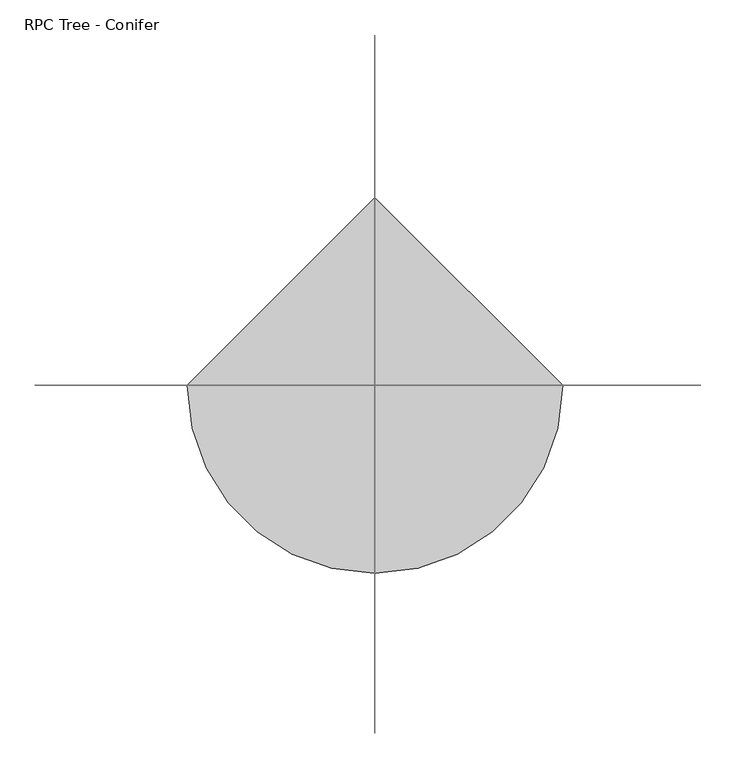
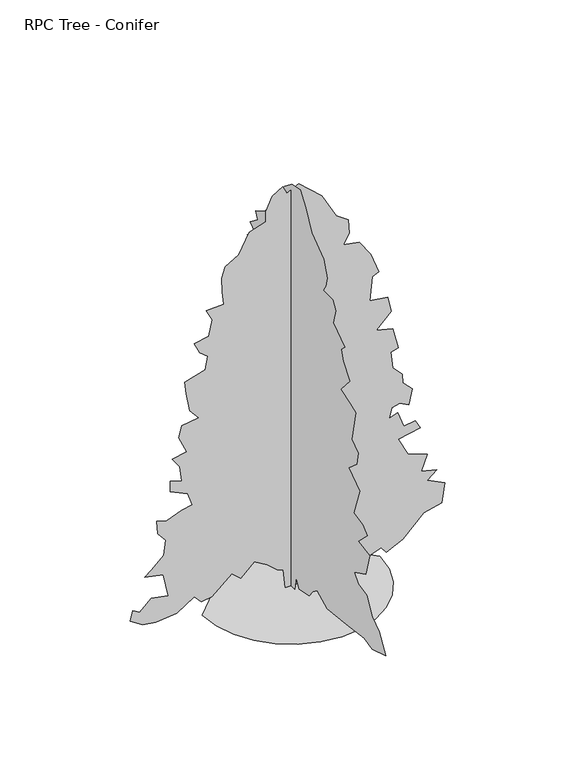
"""IFC4 building model written with IfcOpenShell, lengths in millimetres: geographic element geometry, RPC Tree - Conifer : Colorado Spruce - 4.0 Meters."""

from ifc_helpers import new_model, si_unit, origin, place, context, project, spatial, triangles, source, transform, mapped, element, save


def rpc_tree_conifer_422bf689(model_context):
    return source(origin(), model_context, "Body", "Tessellation", [
        triangles([(0.1966733, 49.8245024, 3.62e-05), (0.1966808, 76.8972503, 209.81401), (0.1966851, 110.7382534, 304.5675106), (0.1966885, 232.5655101, 236.886758), (0.1966934, 381.4650152, 175.9729979), (0.1967001, 550.6700214, 148.90025), (0.1967079, 720.3449844, 156.1022449), (0.1967054, 740.1800383, 40.6092491), (0.1967132, 862.0074858, 121.827502), (0.1967165, 991.2750315, 36.3350005), (0.1967216, 1085.3575155, 67.6820016), (0.1967296, 1268.1000675, 60.913751), (0.1967359, 1356.0849586, 142.1320039), (0.1967499, 1545.5950481, 324.872503), (0.1967463, 1430.5350655, 379.0174902), (0.1967428, 1329.0124832, 412.8600102), (0.1967383, 1234.4449997, 404.9600201), (0.1967407, 1213.9525005, 514.3825198), (0.1967447, 1241.024976, 609.1374919), (0.1967522, 1335.779948, 717.4275026), (0.1967485, 1241.024976, 737.7325132), (0.1967539, 1315.4749374, 805.4150099), (0.1967498, 1200.4174982, 839.2550228), (0.1967461, 1078.589978, 900.169982), (0.1967471, 1015.9549931, 1025.5049915), (0.1967554, 1173.3450228, 1069.3749882), (0.1967602, 1241.024976, 1130.2874765), (0.1967569, 1153.0400122, 1150.5924871), (0.1967529, 1004.1400166, 1238.5800671), (0.1967593, 1112.429991, 1292.7250179), (0.196765, 1121.189994, 1470.9574528), (0.19676, 997.3700083, 1489.0025723), (0.196756, 889.0800339, 1516.0750477), (0.1967604, 905.0550035, 1639.3949913), (0.1967674, 1036.9399767, 1676.5725185), (0.1967726, 1065.0525049, 1807.1075741), (0.1967671, 956.7625305, 1786.8025635), (0.196768, 888.3749897, 1918.5275173), (0.1967741, 963.5299953, 2010.1524479), (0.1967722, 868.7750233, 2091.3700195), (0.1967785, 963.5299953, 2159.0525162), (0.1967813, 990.6025434, 2213.197467), (0.196777, 821.3975372, 2321.4899849), (0.1967781, 801.0925266, 2389.1700108), (0.1967862, 936.4575199, 2456.8526527), (0.1967861, 875.5424881, 2544.8498978), (0.1967818, 740.1800383, 2605.7499596), (0.1967888, 828.1650021, 2707.2751579), (0.1967872, 733.41003, 2795.2500206), (0.1967844, 611.5849806, 2883.2498817), (0.1967873, 604.8150086, 2991.5499573), (0.1967932, 706.3374819, 3038.9249725), (0.1967915, 631.8899912, 3093.0751556), (0.1967882, 543.9025203, 3113.3750793), (0.1967957, 658.9625393, 3194.5750648), (0.1967931, 537.1350191, 3289.3500938), (0.1967966, 570.9749957, 3357.0250328), (0.1967927, 428.8425013, 3438.2500168), (0.1967912, 313.7825186, 3560.0751389), (0.1967925, 237.8634971, 3716.3499023), (0.1967912, 97.2017522, 3884.9500763), (0.196789, -11.0894496, 3972.924939), (0.1967837, -146.4532518, 4000.0000305), (0.1967759, -241.2080059, 3878.1749084), (0.196766, -335.9624874, 3688.6751381), (0.196753, -532.2400054, 3546.5250938), (0.1967459, -586.3849926, 3390.8750015), (0.1967443, -559.3125172, 3296.0999725), (0.196744, -525.4725042, 3235.1999107), (0.1967374, -674.3724998, 3235.1999107), (0.1967328, -721.7499859, 3153.9749268), (0.1967304, -681.1400373, 3011.849881), (0.1967181, -870.6499815, 2883.2498817), (0.1967192, -809.7350224, 2829.0999893), (0.1967147, -843.5775061, 2727.5750816), (0.196706, -951.8674805, 2598.9750824), (0.1967076, -802.9674849, 2429.780032), (0.1966991, -959.7425085, 2380.804969), (0.1966941, -1046.6225252, 2341.7949955), (0.1966879, -985.7074934, 2043.9925335), (0.1966812, -1087.2324738, 1969.542572), (0.1966785, -1066.9275358, 1847.7149792), (0.1966808, -938.3300074, 1732.6574673), (0.1966693, -1114.3050219, 1610.8300198), (0.1966655, -1012.7825123, 1333.3325684), (0.1966581, -1161.6825079, 1306.2599476), (0.1966529, -1236.132542, 1245.3475319), (0.1966552, -1087.2324738, 1096.4475363), (0.1966459, -1276.7399471, 1069.3749882), (0.1966422, -1209.0599939, 846.0224876), (0.1966478, -1026.3175146, 758.0375238), (0.1966426, -1087.2324738, 676.8200249), (0.1966355, -1229.3624611, 649.7474768), (0.1966269, -1317.3499683, 494.0775092), (0.1966194, -1432.409951, 412.8600102), (0.1966096, -1533.9325333, 236.886758), (0.1966172, -1317.3499683, 169.2047519), (0.1966241, -1184.517524, 199.5652534), (0.1966359, -895.4949766, 164.0745054), (0.1966487, -586.3849926, 128.5955028), (0.1966584, -423.9474875, 209.81401), (0.1966598, -356.267498, 155.6682598), (0.1966603, -295.3525025, 81.2182529), (0.1966665, -132.9167506, 47.3774997), (0.1966712, -85.8942484, 133.3167535), (0.1966685, -58.4667483, 3.3e-05), (-51.204578, 1.3e-06, 3.62e-05), (-71.5090799, -2.08e-05, 182.7412439), (-125.6545758, -2.01e-05, 203.0457458), (-220.4093299, -2.09e-05, 284.2650071), (-342.2358327, -2.06e-05, 358.7149867), (-470.8333248, 3.2e-06, 236.886758), (-552.0508238, 2.3e-06, 311.3375007), (-741.5608406, 1.52e-05, 148.90025), (-836.7233459, 1.86e-05, 136.9905027), (-903.9958385, 1.73e-05, 209.81401), (-1066.4333799, 2.7e-05, 101.5230001), (-1262.7108616, 4.83e-05, 81.2184982), (-1384.5383091, 5.1e-05, 101.5230001), (-1499.5984371, 5.11e-05, 175.9729979), (-1479.2934265, 4.63e-05, 270.7274976), (-1411.6109299, 4.61e-05, 230.1184938), (-1303.318412, 2.38e-05, 331.6425113), (-1147.6508789, 2.04e-05, 304.5675106), (-1193.5583965, 1.17e-05, 528.1124957), (-1364.2332985, 1.53e-05, 561.7600059), (-1303.318412, 1.14e-05, 609.1374919), (-1188.2609001, 3.1e-06, 717.4275026), (-1167.9558895, -3.8e-06, 859.5600334), (-1242.405851, -5.5e-06, 947.5475407), (-1255.9433968, -1.09e-05, 1076.1425257), (-1161.188352, -1.25e-05, 1049.0699776), (-1019.0558939, -3.37e-05, 1103.2150011), (-924.3008492, -3.74e-05, 1123.5200117), (-964.9108704, -4.17e-05, 1245.3475319), (-1127.4908449, -4.02e-05, 1321.492448), (-1127.3458683, -4.5e-05, 1428.0875404), (-1019.0558939, -4.67e-05, 1394.2474548), (-1037.3183693, -5.26e-05, 1538.1075691), (-1107.0433285, -5.5e-05, 1637.9024952), (-971.6783352, -6.02e-05, 1664.9749706), (-1046.1283693, -6.53e-05, 1827.4099686), (-1019.0558939, -7.09e-05, 1935.7024864), (-863.3883608, -9.13e-05, 1962.7749619), (-944.6058598, -9.31e-05, 2057.5300793), (-978.4458727, -0.0001002, 2240.2700878), (-991.9833458, -0.000105, 2355.3300705), (-802.473329, -0.0001134, 2416.2424862), (-775.4008535, -0.0001196, 2538.0750206), (-849.8508877, -0.0001201, 2598.9750824), (-903.9958385, -0.0001233, 2707.2751579), (-766.3633965, -0.000143, 2730.4499062), (-734.7908323, -0.0001508, 2883.2498817), (-788.9358559, -0.000154, 2991.5499573), (-626.5008579, -0.0001591, 2998.3001266), (-640.0358603, -0.0001645, 3126.9001259), (-646.8058685, -0.0001703, 3262.2750023), (-612.9633848, -0.0001759, 3363.79991), (-487.5108315, -0.0001976, 3440.9251442), (-389.6133187, -0.0002089, 3627.7500778), (-233.9455858, -0.0002156, 3675.1250931), (-233.9455858, -0.0002202, 3776.6500008), (-173.0318439, -0.0002277, 3905.25), (-78.277326, -0.0002333, 3966.1500618), (-37.6680814, -0.0002312, 3891.699955), (70.622924, -0.0002513, 3945.8501381), (287.2041627, -0.000249, 3749.5749092), (422.5691923, -0.0002276, 3505.9249557), (537.629175, -0.0002419, 3424.6999718), (544.3966762, -0.0002216, 3289.3500938), (490.251689, -0.0002157, 3194.5750648), (639.1516846, -0.000219, 3167.5249718), (747.441659, -0.0002152, 3011.849881), (821.8916204, -0.0002087, 2815.5749428), (760.3216867, -0.0002054, 2783.5501534), (733.9066566, -0.0001945, 2558.3749443), (903.1091194, -0.0001984, 2531.3001434), (936.9516758, -0.0001927, 2382.4025459), (794.819145, -0.0001824, 2247.0400234), (950.4866781, -0.0001853, 2206.4300022), (1004.6341724, -0.000163, 1996.6150475), (930.1816675, -0.0001602, 1983.0799725), (950.4866781, -0.0001535, 1820.6425037), (1039.9941507, -0.0001518, 1722.8699833), (1045.2416502, -0.0001482, 1637.9024952), (1133.2291574, -0.0001468, 1549.9149879), (1099.3866737, -0.0001392, 1401.015065), (1018.1691748, -0.0001389, 1448.392551), (943.7191406, -0.0001358, 1428.0875404), (916.6466652, -0.0001307, 1333.3325684), (997.8641642, -0.0001343, 1360.4050438), (1052.0091877, -0.000129, 1204.7375107), (1160.3016329, -0.0001331, 1225.0425213), (1207.6791189, -0.0001306, 1137.055014), (1004.6341724, -0.0001227, 1096.4475363), (1092.6191362, -0.000103, 920.4725218), (1275.3616882, -0.0001199, 852.7924959), (1216.884153, -9.7e-05, 703.8949711), (1363.3467247, -9.98e-05, 670.0500166), (1275.3616882, -9.39e-05, 595.6000188), (1437.7966862, -9.51e-05, 514.3825198), (1410.7242107, -8.58e-05, 324.872503), (1241.5191319, -7.9e-05, 284.2650071), (1046.1716806, -6.47e-05, 94.2452466), (889.5741171, -4.22e-05, 20.3044996), (842.1966311, -4.35e-05, 81.2182529), (664.5366177, -3.55e-05, 20.9521254), (476.7141795, -2.96e-05, 13.5363501), (402.2641817, -3.04e-05, 81.2182529), (233.0594117, -2.8e-05, 142.1320039), (73.3656708, -2.18e-05, 109.4187482), (57.0864228, -1.64e-05, 3.3e-05), (-828.2308411, -4.6e-06, 5.94e-05), (-806.3283262, -189.8204993, 5.31e-05), (-743.9558252, -364.1400189, 4.6e-05), (-646.1033678, -517.9650046, 3.85e-05), (-517.7683233, -646.3000128, 3.09e-05), (-363.9433376, -744.1524702, 2.34e-05), (-189.6238362, -806.5249712, 1.63e-05), (0.1967073, -828.427486, 1e-05), (190.0171625, -806.5249712, 5e-06), (364.3367002, -744.1524702, 1.7e-06), (518.1616859, -646.3000128, 0.0), (646.4966578, -517.9650046, 0.0), (744.3491152, -364.1400189, 1.7e-06), (806.7216162, -189.8204993, 5e-06), (828.624131, 7.68e-05, 1e-05), (0.1965624, 828.427486, 5.94e-05)], [[26, 27, 28], [21, 22, 23], [19, 20, 21], [51, 52, 53], [7, 8, 9], [35, 36, 37], [13, 14, 15], [34, 35, 37], [54, 55, 56], [72, 73, 74], [95, 96, 97], [88, 89, 90], [44, 45, 46], [86, 87, 88], [85, 86, 88], [51, 53, 54], [44, 46, 47], [88, 90, 91], [13, 15, 16], [13, 16, 17], [38, 39, 40], [25, 26, 28], [25, 28, 29], [47, 48, 49], [56, 57, 58], [30, 31, 32], [29, 30, 32], [41, 42, 43], [40, 41, 43], [106, 1, 2], [105, 106, 2], [75, 76, 77], [94, 95, 97], [94, 97, 98], [78, 79, 80], [83, 84, 85], [29, 32, 33], [103, 104, 105], [12, 13, 17], [11, 12, 17], [77, 78, 80], [102, 103, 105], [62, 63, 64], [80, 81, 82], [80, 82, 83], [61, 62, 64], [61, 64, 65], [60, 61, 65], [59, 60, 65], [69, 70, 71], [69, 71, 72], [94, 98, 99], [93, 94, 99], [92, 93, 99], [92, 99, 100], [91, 92, 100], [91, 100, 101], [47, 49, 50], [9, 10, 11], [9, 11, 17], [9, 17, 18], [7, 9, 18], [59, 65, 66], [59, 66, 67], [59, 67, 68], [59, 68, 69], [58, 59, 69], [56, 58, 69], [54, 56, 69], [54, 69, 72], [51, 54, 72], [50, 51, 72], [50, 72, 74], [50, 74, 75], [50, 75, 77], [47, 50, 77], [44, 47, 77], [43, 44, 77], [40, 43, 77], [40, 77, 80], [40, 80, 83], [38, 40, 83], [38, 83, 85], [37, 38, 85], [34, 37, 85], [33, 34, 85], [29, 33, 85], [25, 29, 85], [25, 85, 88], [25, 88, 91], [25, 91, 101], [25, 101, 102], [24, 25, 102], [23, 24, 102], [21, 23, 102], [105, 2, 3], [102, 105, 3], [21, 102, 3], [21, 3, 4], [21, 4, 5], [21, 5, 6], [21, 6, 7], [21, 7, 18], [19, 21, 18], [125, 126, 127], [198, 199, 200], [153, 154, 155], [139, 140, 141], [130, 131, 132], [120, 121, 122], [119, 120, 122], [186, 187, 188], [136, 137, 138], [135, 136, 138], [150, 151, 152], [193, 194, 195], [192, 193, 195], [125, 127, 128], [180, 181, 182], [163, 164, 165], [185, 186, 188], [196, 197, 198], [190, 191, 192], [111, 112, 113], [212, 107, 108], [211, 212, 108], [173, 174, 175], [149, 150, 152], [179, 180, 182], [129, 130, 132], [146, 147, 148], [204, 205, 206], [200, 201, 202], [200, 202, 203], [162, 163, 165], [190, 192, 195], [165, 166, 167], [118, 119, 122], [118, 122, 123], [118, 123, 124], [117, 118, 124], [116, 117, 124], [176, 177, 178], [176, 178, 179], [129, 132, 133], [185, 188, 189], [142, 143, 144], [141, 142, 144], [161, 162, 165], [161, 165, 167], [161, 167, 168], [116, 124, 125], [145, 146, 148], [144, 145, 148], [114, 115, 116], [113, 114, 116], [113, 116, 125], [113, 125, 128], [113, 128, 129], [113, 129, 133], [113, 133, 134], [111, 113, 134], [168, 169, 170], [168, 170, 171], [161, 168, 171], [160, 161, 171], [159, 160, 171], [158, 159, 171], [157, 158, 171], [156, 157, 171], [155, 156, 171], [171, 172, 173], [171, 173, 175], [155, 171, 175], [155, 175, 176], [153, 155, 176], [152, 153, 176], [149, 152, 176], [149, 176, 179], [148, 149, 179], [144, 148, 179], [144, 179, 182], [144, 182, 183], [141, 144, 183], [139, 141, 183], [138, 139, 183], [135, 138, 183], [134, 135, 183], [111, 134, 183], [110, 111, 183], [110, 183, 184], [110, 184, 185], [110, 185, 189], [110, 189, 190], [110, 190, 195], [109, 110, 195], [108, 109, 195], [211, 108, 195], [210, 211, 195], [210, 195, 196], [209, 210, 196], [209, 196, 198], [208, 209, 198], [207, 208, 198], [206, 207, 198], [204, 206, 198], [203, 204, 198], [200, 203, 198], [227, 228, 213], [226, 227, 213], [226, 213, 214], [225, 226, 214], [225, 214, 215], [225, 215, 216], [224, 225, 216], [223, 224, 216], [223, 216, 217], [223, 217, 218], [223, 218, 219], [223, 219, 220], [223, 220, 221], [223, 221, 222]], closed=False),
    ])


if __name__ == "__main__":
    model = new_model("IFC4")
    model_context = context("Model", 3, world=origin())
    ifc_project = project(units=[si_unit("LENGTHUNIT", "METRE", prefix="MILLI")], contexts=[model_context])
    site = spatial("IfcSite", under=ifc_project)
    building = spatial("IfcBuilding", under=site)
    placement = place(None, origin())
    rpc_tree_conifer_shape = rpc_tree_conifer_422bf689(model_context)
    element("IfcGeographicElement", 1, ObjectType="RPC Tree - Conifer : Colorado Spruce - 4.0 Meters", at=placement, inside=building, context=model_context, shape_type="MappedRepresentation", body=[
        mapped(rpc_tree_conifer_shape, transform((0.0, 0.0, 0.0), x_axis=(1.0, 0.0, 0.0), y_axis=(0.0, 1.0, 0.0), z_axis=(0.0, 0.0, 1.0))),
    ])
    save(model, "model.ifc")

# Revit data of these elements
# Type "RPC Tree - Conifer : Colorado Spruce - 4.0 Meters"
#   built-in parameter 1005198 = "{2, 15},{39, RPC-16-G0M4-N9PX-U6TN-C000-ST1L-LVER-AU},{1, 0},{1, 0},{2, 13},{1, 8},{5, Color},{1, 0},{1, 0},{3, 0.8},{3, 0.8},{3, 0.8},{1, 8},{7, BBoxMin},{1, 0},{1, 0},{1, 0},{1, 0},{1, 0},{1, 8},{7, BBoxMax},{1, 0},{1, 0},{1, 0},{1, 0},{1, 0},{2, 11},{9, RPCTypeId},{1, 0},{1, 0},{39, RPC-16-G0M4-N9PX-U6TN-C000-ST1L-LVER-AU},{1, 6},{14, RPCPlantHeight},{1, 0},{1, 0},{7, 13.1234},{2, 11},{7, keyword},{1, 0},{1, 0},{34, :RPCs:Trees [General]:Geometry:RPC},{2, 11},{8, category},{1, 0},{1, 0},{15, Trees [General]},{2, 11},{12, LocalizedUID},{1, 0},{1, 0},{15, Colorado Spruce},{2, 14},{6, Height},{1, 0},{1, 0},{7, 13.1234},{1, 2},{16, Cast Reflections},{1, 0},{1, 0},{1, 0},{1, 2},{12, Cast Shadows},{1, 0},{1, 0},{1, 1},{1, 2},{9, Lock View},{1, 0},{1, 0},{1, 0},{1, 4},{5, ViewC},{1, 0},{1, 0},{1, 0},{21, assetlibrary_base.fbx},{1, 5},"
#   built-in parameter 1005195 = "RPC-16-G0M4-N9PX-U6TN-C000-ST1L-LVER-AU"
#   Type Comments = "Colorado Spruce"
#   Height = 4000 mm
#   Description = (empty or 0)
